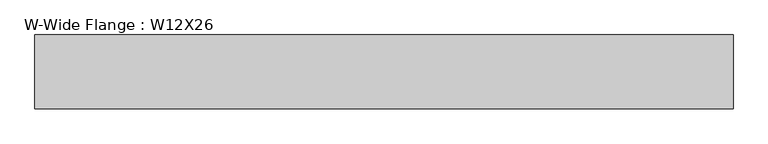
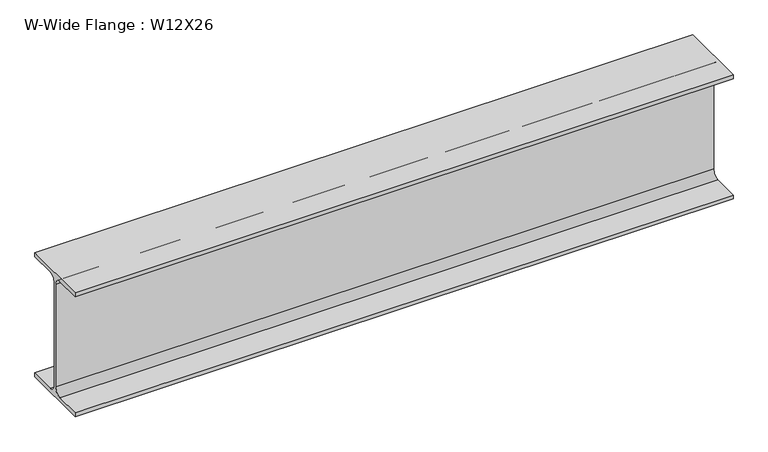
"""IFC4 building model written with IfcOpenShell, lengths in millimetres: beam geometry, W-Wide Flange : W12X26."""

import ifcopenshell
import ifcopenshell.guid

model = None  # the IFC model being written
_history = None  # IfcOwnerHistory: only IFC2X3 demands one
_inside = {}  # id of a spatial element -> (the spatial element, [elements in it])
_under = {}  # id of a project, library or spatial element -> (it, [spatial elements below it])
_declared = {}  # id of a project -> (the project, [libraries it declares])
_typed = {}  # id of a type object -> (the type object, [elements of that type])
_made_of = {}  # id of a material, layer set ... -> (it, [elements and type objects made of it])


def new_model(schema):
    """Start an empty IFC model of exactly this schema.

    Asked for "IFC4X3", IfcOpenShell would pick the latest addendum, in which some entities
    have other attributes; the version numbers below select the first issue.
    IFC2X3 requires an IfcOwnerHistory on every rooted entity: one is made here for all.
    """
    global model, _history
    if schema == "IFC4X3":
        model = ifcopenshell.file(schema_version=(4, 3, 0, 0))
    else:
        model = ifcopenshell.file(schema=schema)
    _inside.clear()
    _under.clear()
    _declared.clear()
    _typed.clear()
    _made_of.clear()
    _history = None
    if model.schema == "IFC2X3":
        org = make("IfcOrganization", Name="unknown")
        user = make(
            "IfcPersonAndOrganization",
            ThePerson=make("IfcPerson", FamilyName="unknown"),
            TheOrganization=org,
        )
        app = make(
            "IfcApplication",
            ApplicationDeveloper=org,
            Version="unknown",
            ApplicationFullName="unknown",
            ApplicationIdentifier="unknown",
        )
        _history = make(
            "IfcOwnerHistory",
            OwningUser=user,
            OwningApplication=app,
            ChangeAction="ADDED",
            CreationDate=0,
        )
    return model


def make(cls, **values):
    """One entity of the class cls with the attributes given. An attribute that is None is left unset."""
    return model.create_entity(
        cls, **{name: value for name, value in values.items() if value is not None}
    )


def rooted(cls, **values):
    """An entity with a GlobalId (a new one), such as an element, a storey or a relation."""
    return make(cls, GlobalId=ifcopenshell.guid.new(), OwnerHistory=_history, **values)


def si_unit(unit_type, name, prefix=None):
    """IfcSIUnit, for example si_unit("LENGTHUNIT", "METRE", prefix="MILLI")."""
    return make("IfcSIUnit", UnitType=unit_type, Prefix=prefix, Name=name)


def assignment(units):
    """IfcUnitAssignment: the units of a project."""
    return None if units is None else make("IfcUnitAssignment", Units=units)


def point(xyz):
    """IfcCartesianPoint."""
    return None if xyz is None else make("IfcCartesianPoint", Coordinates=xyz)


def direction(xyz):
    """IfcDirection."""
    return None if xyz is None else make("IfcDirection", DirectionRatios=xyz)


def frame(location, z_axis=None, x_axis=None):
    """IfcAxis2Placement3D, a coordinate frame: its origin and axes. An axis left out is left unset."""
    return make(
        "IfcAxis2Placement3D",
        Location=point(location),
        Axis=direction(z_axis),
        RefDirection=direction(x_axis),
    )


def frame_2d(location, x_axis=None):
    """IfcAxis2Placement2D, a coordinate frame in the plane: its origin and x axis."""
    return make(
        "IfcAxis2Placement2D", Location=point(location), RefDirection=direction(x_axis)
    )


def origin():
    """The frame at (0, 0, 0) with its axes left unset."""
    return frame((0.0, 0.0, 0.0))


def place(relative_to, where):
    """IfcLocalPlacement: puts the frame where relative to a parent placement (None: the world)."""
    return make(
        "IfcLocalPlacement", PlacementRelTo=relative_to, RelativePlacement=where
    )


def context(
    kind, dimensions, precision=None, world=None, true_north=None, identifier=None
):
    """IfcGeometricRepresentationContext, for example the 3D "Model" context."""
    return make(
        "IfcGeometricRepresentationContext",
        ContextIdentifier=identifier,
        ContextType=kind,
        CoordinateSpaceDimension=dimensions,
        Precision=precision,
        WorldCoordinateSystem=world,
        TrueNorth=true_north,
    )


def project(units=None, contexts=None):
    """IfcProject with its units and contexts."""
    return rooted(
        "IfcProject",
        Name="project",
        RepresentationContexts=contexts,
        UnitsInContext=assignment(units),
    )


def spatial(cls, under=None, at=None, **own):
    """A site, building, storey or space (cls), placed at a placement, below another one or the project."""
    s = rooted(cls, ObjectPlacement=at, **own)
    if under is not None:
        _under.setdefault(under.id(), (under, []))[1].append(s)
    return s


def polyline(points):
    """IfcPolyline through the points."""
    return make("IfcPolyline", Points=[point(p) for p in points])


def circle_curve(where, radius):
    """IfcCircle in the frame where."""
    return make("IfcCircle", Position=where, Radius=radius)


def trimmed(basis, trim1, trim2, sense, master):
    """IfcTrimmedCurve: the piece of a basis curve between two trims."""
    return make(
        "IfcTrimmedCurve",
        BasisCurve=basis,
        Trim1=trim1,
        Trim2=trim2,
        SenseAgreement=sense,
        MasterRepresentation=master,
    )


def segment(curve, same_sense, transition):
    """IfcCompositeCurveSegment."""
    return make(
        "IfcCompositeCurveSegment",
        Transition=transition,
        SameSense=same_sense,
        ParentCurve=curve,
    )


def composite_curve(segments, self_intersect=None):
    """IfcCompositeCurve: segments joined end to end."""
    return make("IfcCompositeCurve", Segments=segments, SelfIntersect=self_intersect)


def outline(outer, holes=None, kind="AREA"):
    """IfcArbitraryClosedProfileDef: a profile drawn as a closed curve; with holes, ...WithVoids."""
    if holes is None:
        return make("IfcArbitraryClosedProfileDef", ProfileType=kind, OuterCurve=outer)
    return make(
        "IfcArbitraryProfileDefWithVoids",
        ProfileType=kind,
        OuterCurve=outer,
        InnerCurves=holes,
    )


def extrude(swept, where, along, depth):
    """IfcExtrudedAreaSolid: the profile swept, set in the frame where, extruded along a direction by depth."""
    return make(
        "IfcExtrudedAreaSolid",
        SweptArea=swept,
        Position=where,
        ExtrudedDirection=direction(along),
        Depth=depth,
    )


def shape(context_of_items, identifier, shape_type, items):
    """IfcShapeRepresentation: the items that make up one representation, for example the "Body"."""
    return make(
        "IfcShapeRepresentation",
        ContextOfItems=context_of_items,
        RepresentationIdentifier=identifier,
        RepresentationType=shape_type,
        Items=items,
    )


def source(mapping_origin, context_of_items, identifier, shape_type, items):
    """IfcRepresentationMap: a shape defined once, which mapped items show again and again."""
    return make(
        "IfcRepresentationMap",
        MappingOrigin=mapping_origin,
        MappedRepresentation=shape(context_of_items, identifier, shape_type, items),
    )


def transform(
    local_origin,
    x_axis=None,
    y_axis=None,
    z_axis=None,
    scale=None,
    scale2=None,
    scale3=None,
    uniform=True,
):
    """IfcCartesianTransformationOperator3D, or its non-uniform kind. x_axis, y_axis, z_axis: its Axis1, 2, 3."""
    if uniform:
        return make(
            "IfcCartesianTransformationOperator3D",
            Axis1=direction(x_axis),
            Axis2=direction(y_axis),
            LocalOrigin=point(local_origin),
            Scale=scale,
            Axis3=direction(z_axis),
        )
    return make(
        "IfcCartesianTransformationOperator3DnonUniform",
        Axis1=direction(x_axis),
        Axis2=direction(y_axis),
        LocalOrigin=point(local_origin),
        Scale=scale,
        Axis3=direction(z_axis),
        Scale2=scale2,
        Scale3=scale3,
    )


def mapped(mapping_source, mapping_target):
    """IfcMappedItem: shows the shape of a source again, moved by a transform."""
    return make(
        "IfcMappedItem", MappingSource=mapping_source, MappingTarget=mapping_target
    )


def made_of(thing, what):
    """Note that an element or type object is made of a material, layer set ...; save() writes the relation."""
    if what is not None:
        _made_of.setdefault(what.id(), (what, []))[1].append(thing)
    return thing


def element(
    cls,
    number,
    at=None,
    inside=None,
    cuts=None,
    type_object=None,
    material=None,
    context=None,
    identifier="Body",
    shape_type=None,
    held_by="IfcProductDefinitionShape",
    body=None,
    shapes=None,
    **own,
):
    """One element of the class cls, such as IfcWall. Its Tag is "e" and its number.

    at: its placement. inside: the storey or other place that contains it. cuts: it is an
    opening in that element (IfcRelVoidsElement). A single representation is given by context,
    identifier, shape_type and body (its items); several are given by shapes. held_by: the class
    of the entity that holds the representations. save() writes the other relations.
    """
    e = rooted(cls, Tag="e%d" % number, ObjectPlacement=at, **own)
    if body is not None:
        shapes = [shape(context, identifier, shape_type, body)]
    if shapes is not None:
        e.Representation = make(held_by, Representations=shapes)
    if inside is not None:
        _inside.setdefault(inside.id(), (inside, []))[1].append(e)
    if cuts is not None:
        rooted(
            "IfcRelVoidsElement", RelatingBuildingElement=cuts, RelatedOpeningElement=e
        )
    if type_object is not None:
        _typed.setdefault(type_object.id(), (type_object, []))[1].append(e)
    return made_of(e, material)


def aggregate(whole, parts):
    """IfcRelAggregates: a whole, such as a stair, and the parts it consists of."""
    return rooted("IfcRelAggregates", RelatingObject=whole, RelatedObjects=parts)


def save(model, path):
    """Write the relations noted so far, then the file.

    IfcRelAggregates (storeys below a building ...), IfcRelContainedInSpatialStructure (elements
    in a storey), IfcRelDefinesByType, IfcRelAssociatesMaterial and IfcRelDeclares: one each for
    every whole, place, type object, material and project.
    """
    for whole, parts in _under.values():
        aggregate(whole, parts)
    for where, things in _inside.values():
        rooted(
            "IfcRelContainedInSpatialStructure",
            RelatedElements=things,
            RelatingStructure=where,
        )
    for kind, things in _typed.values():
        rooted("IfcRelDefinesByType", RelatedObjects=things, RelatingType=kind)
    for what, things in _made_of.values():
        rooted("IfcRelAssociatesMaterial", RelatedObjects=things, RelatingMaterial=what)
    for by, libraries in _declared.values():
        rooted("IfcRelDeclares", RelatingContext=by, RelatedDefinitions=libraries)
    model.write(path)


def w_wide_flange_w12x26_481373e5(model_context):
    return source(origin(), model_context, "Body", "SweptSolid", [
        extrude(outline(composite_curve([segment(polyline([(82.4011719, -145.5539063), (82.4011719, -155.178125), (-82.4011719, -155.178125), (-82.4011719, -145.5539063), (-20.2902344, -145.5539063)]), True, "CONTINUOUS"), segment(trimmed(circle_curve(frame_2d((-20.2902344, -128.190625)), 17.3632812), [point((-20.2902344, -145.5539063))], [point((-2.9269531, -128.190625))], True, "CARTESIAN"), True, "CONTINUOUS"), segment(polyline([(-2.9269531, -128.190625), (-2.9269531, 128.190625)]), True, "CONTINUOUS"), segment(trimmed(circle_curve(frame_2d((-20.2902344, 128.190625)), 17.3632812), [point((-2.9269531, 128.190625))], [point((-20.2902344, 145.5539062))], True, "CARTESIAN"), True, "CONTINUOUS"), segment(polyline([(-20.2902344, 145.5539062), (-82.4011719, 145.5539062), (-82.4011719, 155.178125), (82.4011719, 155.178125), (82.4011719, 145.5539062), (20.2902344, 145.5539062)]), True, "CONTINUOUS"), segment(trimmed(circle_curve(frame_2d((20.2902344, 128.190625)), 17.3632812), [point((20.2902344, 145.5539062))], [point((2.9269531, 128.190625))], True, "CARTESIAN"), True, "CONTINUOUS"), segment(polyline([(2.9269531, 128.190625), (2.9269531, -128.190625)]), True, "CONTINUOUS"), segment(trimmed(circle_curve(frame_2d((20.2902344, -128.190625)), 17.3632812), [point((2.9269531, -128.190625))], [point((20.2902344, -145.5539063))], True, "CARTESIAN"), True, "CONTINUOUS"), segment(polyline([(20.2902344, -145.5539063), (82.4011719, -145.5539063)]), True, "CONTINUOUS")], self_intersect=False)), frame((-783.4151988, 0.0, 0.0), z_axis=(1.0, 0.0, 0.0), x_axis=(0.0, 1.0, 0.0)), (0.0, 0.0, 1.0), 1557.6384395),
    ])


if __name__ == "__main__":
    model = new_model("IFC4")
    model_context = context("Model", 3, world=origin())
    ifc_project = project(units=[si_unit("LENGTHUNIT", "METRE", prefix="MILLI")], contexts=[model_context])
    site = spatial("IfcSite", under=ifc_project)
    building = spatial("IfcBuilding", under=site)
    placement = place(None, origin())
    w_wide_flange_w12x26_shape = w_wide_flange_w12x26_481373e5(model_context)
    element("IfcBeam", 1, ObjectType="W-Wide Flange : W12X26", at=placement, inside=building, context=model_context, shape_type="MappedRepresentation", body=[
        mapped(w_wide_flange_w12x26_shape, transform((0.0, 0.0, 0.0), x_axis=(1.0, 0.0, 0.0), y_axis=(0.0, 1.0, 0.0), z_axis=(0.0, 0.0, 1.0))),
    ])
    save(model, "model.ifc")

# Revit data of these elements
# Type "W-Wide Flange : W12X26"
#   Assembly Code = "B10"
#   Start Extension Calculation [instance default] = 10' - 0"
#   Start Extension [instance default] = -0' - 0 1/2"
#   End Extension Calculation [instance default] = 10' - 0"
#   End Extension [instance default] = -0' - 0 1/2"
#   A = 0.053125 SF
#   Length [instance default] = 5' - 0"
#   W = 26
#   bf = 0' - 6 125/256"
#   d = 1' - 0 7/32"
#   k = 0' - 1 1/16"
#   k2 = 0' - 0 175/256"
#   tf = 0' - 0 97/256"
#   tw = 0' - 0 59/256"
#   Beam Material [instance default] = Metal - Steel - ASTM A992
# Element 1 (IfcBeam, "W-Wide Flange : W12X26")
#   Materials on its faces: "Metal - Steel - ASTM A992"
# Materials
#   "Metal - Steel - ASTM A992": class "Metal", colour RGB 199 199 199, transparency 0
